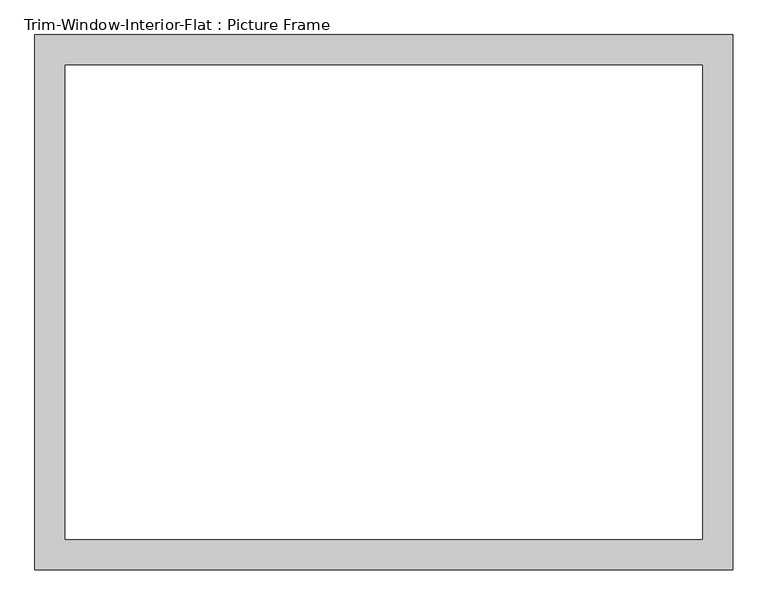
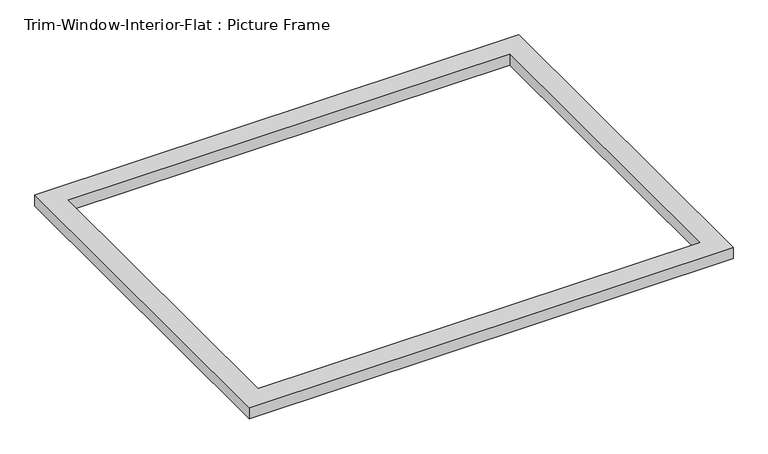
"""IFC4 building model written with IfcOpenShell, lengths in millimetres: proxy geometry, Trim-Window-Interior-Flat : Picture Frame."""

import ifcopenshell
import ifcopenshell.guid

model = None  # the IFC model being written
_history = None  # IfcOwnerHistory: only IFC2X3 demands one
_inside = {}  # id of a spatial element -> (the spatial element, [elements in it])
_under = {}  # id of a project, library or spatial element -> (it, [spatial elements below it])
_declared = {}  # id of a project -> (the project, [libraries it declares])
_typed = {}  # id of a type object -> (the type object, [elements of that type])
_made_of = {}  # id of a material, layer set ... -> (it, [elements and type objects made of it])


def new_model(schema):
    """Start an empty IFC model of exactly this schema.

    Asked for "IFC4X3", IfcOpenShell would pick the latest addendum, in which some entities
    have other attributes; the version numbers below select the first issue.
    IFC2X3 requires an IfcOwnerHistory on every rooted entity: one is made here for all.
    """
    global model, _history
    if schema == "IFC4X3":
        model = ifcopenshell.file(schema_version=(4, 3, 0, 0))
    else:
        model = ifcopenshell.file(schema=schema)
    _inside.clear()
    _under.clear()
    _declared.clear()
    _typed.clear()
    _made_of.clear()
    _history = None
    if model.schema == "IFC2X3":
        org = make("IfcOrganization", Name="unknown")
        user = make(
            "IfcPersonAndOrganization",
            ThePerson=make("IfcPerson", FamilyName="unknown"),
            TheOrganization=org,
        )
        app = make(
            "IfcApplication",
            ApplicationDeveloper=org,
            Version="unknown",
            ApplicationFullName="unknown",
            ApplicationIdentifier="unknown",
        )
        _history = make(
            "IfcOwnerHistory",
            OwningUser=user,
            OwningApplication=app,
            ChangeAction="ADDED",
            CreationDate=0,
        )
    return model


def make(cls, **values):
    """One entity of the class cls with the attributes given. An attribute that is None is left unset."""
    return model.create_entity(
        cls, **{name: value for name, value in values.items() if value is not None}
    )


def rooted(cls, **values):
    """An entity with a GlobalId (a new one), such as an element, a storey or a relation."""
    return make(cls, GlobalId=ifcopenshell.guid.new(), OwnerHistory=_history, **values)


def si_unit(unit_type, name, prefix=None):
    """IfcSIUnit, for example si_unit("LENGTHUNIT", "METRE", prefix="MILLI")."""
    return make("IfcSIUnit", UnitType=unit_type, Prefix=prefix, Name=name)


def assignment(units):
    """IfcUnitAssignment: the units of a project."""
    return None if units is None else make("IfcUnitAssignment", Units=units)


def point(xyz):
    """IfcCartesianPoint."""
    return None if xyz is None else make("IfcCartesianPoint", Coordinates=xyz)


def direction(xyz):
    """IfcDirection."""
    return None if xyz is None else make("IfcDirection", DirectionRatios=xyz)


def frame(location, z_axis=None, x_axis=None):
    """IfcAxis2Placement3D, a coordinate frame: its origin and axes. An axis left out is left unset."""
    return make(
        "IfcAxis2Placement3D",
        Location=point(location),
        Axis=direction(z_axis),
        RefDirection=direction(x_axis),
    )


def origin():
    """The frame at (0, 0, 0) with its axes left unset."""
    return frame((0.0, 0.0, 0.0))


def origin_with_axes():
    """The frame at (0, 0, 0) with the z axis (0, 0, 1) and the x axis (1, 0, 0) written out."""
    return frame((0.0, 0.0, 0.0), z_axis=(0.0, 0.0, 1.0), x_axis=(1.0, 0.0, 0.0))


def place(relative_to, where):
    """IfcLocalPlacement: puts the frame where relative to a parent placement (None: the world)."""
    return make(
        "IfcLocalPlacement", PlacementRelTo=relative_to, RelativePlacement=where
    )


def context(
    kind, dimensions, precision=None, world=None, true_north=None, identifier=None
):
    """IfcGeometricRepresentationContext, for example the 3D "Model" context."""
    return make(
        "IfcGeometricRepresentationContext",
        ContextIdentifier=identifier,
        ContextType=kind,
        CoordinateSpaceDimension=dimensions,
        Precision=precision,
        WorldCoordinateSystem=world,
        TrueNorth=true_north,
    )


def project(units=None, contexts=None):
    """IfcProject with its units and contexts."""
    return rooted(
        "IfcProject",
        Name="project",
        RepresentationContexts=contexts,
        UnitsInContext=assignment(units),
    )


def spatial(cls, under=None, at=None, **own):
    """A site, building, storey or space (cls), placed at a placement, below another one or the project."""
    s = rooted(cls, ObjectPlacement=at, **own)
    if under is not None:
        _under.setdefault(under.id(), (under, []))[1].append(s)
    return s


def polyline(points):
    """IfcPolyline through the points."""
    return make("IfcPolyline", Points=[point(p) for p in points])


def outline(outer, holes=None, kind="AREA"):
    """IfcArbitraryClosedProfileDef: a profile drawn as a closed curve; with holes, ...WithVoids."""
    if holes is None:
        return make("IfcArbitraryClosedProfileDef", ProfileType=kind, OuterCurve=outer)
    return make(
        "IfcArbitraryProfileDefWithVoids",
        ProfileType=kind,
        OuterCurve=outer,
        InnerCurves=holes,
    )


def extrude(swept, where, along, depth):
    """IfcExtrudedAreaSolid: the profile swept, set in the frame where, extruded along a direction by depth."""
    return make(
        "IfcExtrudedAreaSolid",
        SweptArea=swept,
        Position=where,
        ExtrudedDirection=direction(along),
        Depth=depth,
    )


def shape(context_of_items, identifier, shape_type, items):
    """IfcShapeRepresentation: the items that make up one representation, for example the "Body"."""
    return make(
        "IfcShapeRepresentation",
        ContextOfItems=context_of_items,
        RepresentationIdentifier=identifier,
        RepresentationType=shape_type,
        Items=items,
    )


def source(mapping_origin, context_of_items, identifier, shape_type, items):
    """IfcRepresentationMap: a shape defined once, which mapped items show again and again."""
    return make(
        "IfcRepresentationMap",
        MappingOrigin=mapping_origin,
        MappedRepresentation=shape(context_of_items, identifier, shape_type, items),
    )


def transform(
    local_origin,
    x_axis=None,
    y_axis=None,
    z_axis=None,
    scale=None,
    scale2=None,
    scale3=None,
    uniform=True,
):
    """IfcCartesianTransformationOperator3D, or its non-uniform kind. x_axis, y_axis, z_axis: its Axis1, 2, 3."""
    if uniform:
        return make(
            "IfcCartesianTransformationOperator3D",
            Axis1=direction(x_axis),
            Axis2=direction(y_axis),
            LocalOrigin=point(local_origin),
            Scale=scale,
            Axis3=direction(z_axis),
        )
    return make(
        "IfcCartesianTransformationOperator3DnonUniform",
        Axis1=direction(x_axis),
        Axis2=direction(y_axis),
        LocalOrigin=point(local_origin),
        Scale=scale,
        Axis3=direction(z_axis),
        Scale2=scale2,
        Scale3=scale3,
    )


def mapped(mapping_source, mapping_target):
    """IfcMappedItem: shows the shape of a source again, moved by a transform."""
    return make(
        "IfcMappedItem", MappingSource=mapping_source, MappingTarget=mapping_target
    )


def made_of(thing, what):
    """Note that an element or type object is made of a material, layer set ...; save() writes the relation."""
    if what is not None:
        _made_of.setdefault(what.id(), (what, []))[1].append(thing)
    return thing


def element(
    cls,
    number,
    at=None,
    inside=None,
    cuts=None,
    type_object=None,
    material=None,
    context=None,
    identifier="Body",
    shape_type=None,
    held_by="IfcProductDefinitionShape",
    body=None,
    shapes=None,
    **own,
):
    """One element of the class cls, such as IfcWall. Its Tag is "e" and its number.

    at: its placement. inside: the storey or other place that contains it. cuts: it is an
    opening in that element (IfcRelVoidsElement). A single representation is given by context,
    identifier, shape_type and body (its items); several are given by shapes. held_by: the class
    of the entity that holds the representations. save() writes the other relations.
    """
    e = rooted(cls, Tag="e%d" % number, ObjectPlacement=at, **own)
    if body is not None:
        shapes = [shape(context, identifier, shape_type, body)]
    if shapes is not None:
        e.Representation = make(held_by, Representations=shapes)
    if inside is not None:
        _inside.setdefault(inside.id(), (inside, []))[1].append(e)
    if cuts is not None:
        rooted(
            "IfcRelVoidsElement", RelatingBuildingElement=cuts, RelatedOpeningElement=e
        )
    if type_object is not None:
        _typed.setdefault(type_object.id(), (type_object, []))[1].append(e)
    return made_of(e, material)


def aggregate(whole, parts):
    """IfcRelAggregates: a whole, such as a stair, and the parts it consists of."""
    return rooted("IfcRelAggregates", RelatingObject=whole, RelatedObjects=parts)


def save(model, path):
    """Write the relations noted so far, then the file.

    IfcRelAggregates (storeys below a building ...), IfcRelContainedInSpatialStructure (elements
    in a storey), IfcRelDefinesByType, IfcRelAssociatesMaterial and IfcRelDeclares: one each for
    every whole, place, type object, material and project.
    """
    for whole, parts in _under.values():
        aggregate(whole, parts)
    for where, things in _inside.values():
        rooted(
            "IfcRelContainedInSpatialStructure",
            RelatedElements=things,
            RelatingStructure=where,
        )
    for kind, things in _typed.values():
        rooted("IfcRelDefinesByType", RelatedObjects=things, RelatingType=kind)
    for what, things in _made_of.values():
        rooted("IfcRelAssociatesMaterial", RelatedObjects=things, RelatingMaterial=what)
    for by, libraries in _declared.values():
        rooted("IfcRelDeclares", RelatingContext=by, RelatedDefinitions=libraries)
    model.write(path)


def trim_window_interior_flat_picture_frame_cf1733af(model_context):
    return source(origin(), model_context, "Body", "SweptSolid", [
        extrude(outline(polyline([(654.05, 44.45), (654.05, -958.85), (-654.05, -958.85), (-654.05, 44.45), (654.05, 44.45)]), holes=[polyline([(596.9, -12.7), (-596.9, -12.7), (-596.9, -901.7), (596.9, -901.7), (596.9, -12.7)])]), origin_with_axes(), (0.0, 0.0, 1.0), 31.75),
    ])


if __name__ == "__main__":
    model = new_model("IFC4")
    model_context = context("Model", 3, world=origin())
    ifc_project = project(units=[si_unit("LENGTHUNIT", "METRE", prefix="MILLI")], contexts=[model_context])
    site = spatial("IfcSite", under=ifc_project)
    building = spatial("IfcBuilding", under=site)
    placement = place(None, origin())
    trim_window_interior_flat_picture_frame_shape = trim_window_interior_flat_picture_frame_cf1733af(model_context)
    element("IfcBuildingElementProxy", 1, Name="Trim-Window-Interior-Flat : Picture Frame", ObjectType="Trim-Window-Interior-Flat : Picture Frame", at=placement, inside=building, context=model_context, shape_type="MappedRepresentation", body=[
        mapped(trim_window_interior_flat_picture_frame_shape, transform((0.0, 0.0, 0.0), x_axis=(1.0, 0.0, 0.0), y_axis=(0.0, 1.0, 0.0), z_axis=(0.0, 0.0, 1.0))),
    ])
    save(model, "model.ifc")

# Revit data of these elements
# Type "Trim-Window-Interior-Flat : Picture Frame"
#   Trim Thickness_Picture Frame = 0' - 1 1/4"
#   Trim Width = 0' - 2 1/4"
#   Trim Thickness_with Sill = 0' - 0 3/4"
#   Sill Thickness = 0' - 1 1/4"
#   Opening Width [instance default] = 2' - 0"
#   Opening Height [instance default] = 3' - 0"
#   Default Elevation = 4' - 0"
#   Sill = no
#   Picture Frame = yes
#   Trim Material [instance default] = none
# Element 1 (IfcBuildingElementProxy, "Trim-Window-Interior-Flat : Picture Frame")
#   Opening Width = 4' - 0"
#   Trim Material = accent 2
#   Materials on its faces: "accent 2"
# Materials
#   "accent 2": class "Wood", colour RGB 80 80 80, transparency 0, Description = "Wood framing, thermal airspace", Cost = 0
